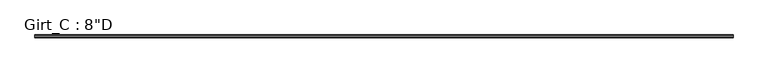
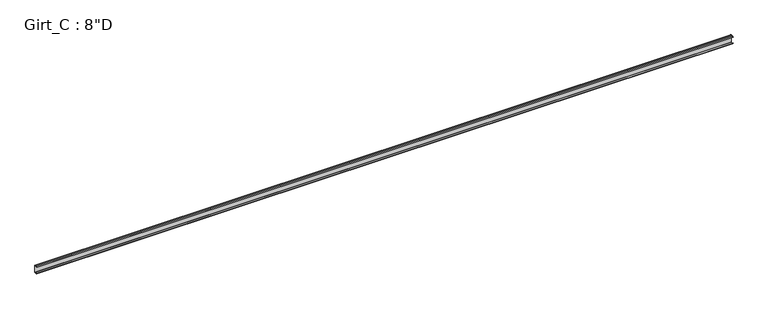
"""IFC4 building model written with IfcOpenShell, lengths in millimetres: beam geometry."""

from ifc_helpers import new_model, si_unit, point, frame, frame_2d, origin, place, context, project, spatial, polyline, circle_curve, trimmed, segment, composite_curve, outline, extrude, source, transform, mapped, element, save


def beam_7a52cf56(model_context):
    return source(origin(), model_context, "Body", "SweptSolid", [
        extrude(outline(composite_curve([segment(polyline([(-63.5, 101.6), (-3.3734375, 101.6)]), True, "CONTINUOUS"), segment(trimmed(circle_curve(frame_2d((-3.3734375, 96.8375)), 4.7625), [point((-3.3734375, 101.6))], [point((1.3890625, 96.8375))], False, "CARTESIAN"), True, "CONTINUOUS"), segment(polyline([(1.3890625, 96.8375), (1.3890625, -96.8375)]), True, "CONTINUOUS"), segment(trimmed(circle_curve(frame_2d((-3.3734375, -96.8375)), 4.7625), [point((1.3890625, -96.8375))], [point((-3.3734375, -101.6))], False, "CARTESIAN"), True, "CONTINUOUS"), segment(polyline([(-3.3734375, -101.6), (-63.5, -101.6), (-75.745104, -87.0068534), (-73.6169367, -85.221109), (-62.204539, -98.821875), (-3.2694106, -98.821875)]), True, "CONTINUOUS"), segment(trimmed(circle_curve(frame_2d((-3.3748024, -96.8389339)), 1.9857399), [point((-3.2694106, -98.821875))], [point((-1.3890625, -96.8389339))], True, "CARTESIAN"), True, "CONTINUOUS"), segment(polyline([(-1.3890625, -96.8389339), (-1.3890625, 96.8381931)]), True, "CONTINUOUS"), segment(trimmed(circle_curve(frame_2d((-3.3741066, 96.8381931)), 1.9850441), [point((-1.3890625, 96.8381931))], [point((-3.3005807, 98.821875))], True, "CARTESIAN"), True, "CONTINUOUS"), segment(polyline([(-3.3005807, 98.821875), (-62.204539, 98.821875), (-73.6169367, 85.221109), (-75.745104, 87.0068534), (-63.5, 101.6)]), True, "CONTINUOUS")], self_intersect=False)), frame((-9148.7289502, 0.0, 0.0), z_axis=(1.0, 0.0, 0.0), x_axis=(0.0, 1.0, 0.0)), (0.0, 0.0, 1.0), 18297.4579005),
    ])


if __name__ == "__main__":
    model = new_model("IFC4")
    model_context = context("Model", 3, world=origin())
    ifc_project = project(units=[si_unit("LENGTHUNIT", "METRE", prefix="MILLI")], contexts=[model_context])
    site = spatial("IfcSite", under=ifc_project)
    building = spatial("IfcBuilding", under=site)
    placement = place(None, origin())
    beam_shape = beam_7a52cf56(model_context)
    element("IfcBeam", 1, ObjectType="Girt_C : 8\"D", at=placement, inside=building, context=model_context, shape_type="MappedRepresentation", body=[
        mapped(beam_shape, transform((0.0, 0.0, 0.0), x_axis=(1.0, 0.0, 0.0), y_axis=(0.0, 1.0, 0.0), z_axis=(0.0, 0.0, 1.0))),
    ])
    save(model, "model.ifc")

# Revit data of these elements
# Type "Girt_C : 8\"D"
#   Web_Thickness = 0' - 0 7/64"
#   Length [instance default] = 10' - 0"
#   Leg_1 = 0' - 2 1/2"
#   Height = 0' - 8"
#   Structural Material [instance default] = none
